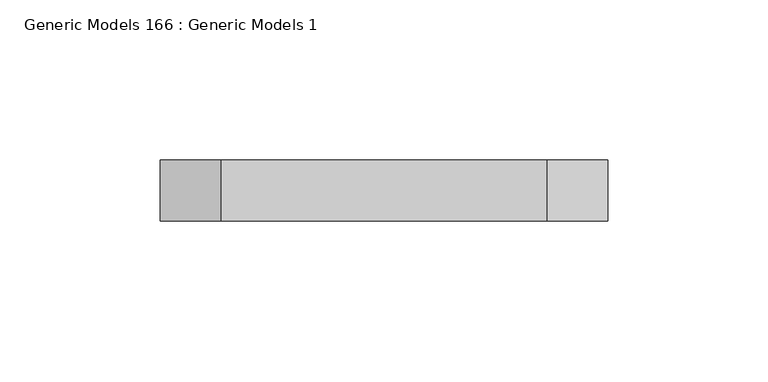
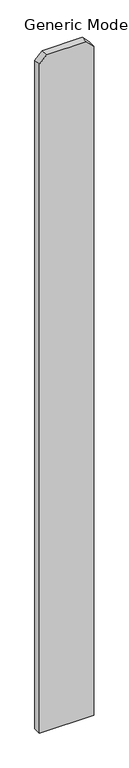
"""IFC4 building model written with IfcOpenShell, lengths in millimetres: proxy geometry, Generic Models 166 : Generic Models 1."""

from ifc_helpers import new_model, si_unit, frame, origin, place, context, project, spatial, polyline, outline, extrude, source, transform, mapped, element, save


def generic_models_166_generic_models_1_bb9aeded(model_context):
    return source(origin(), model_context, "Body", "SweptSolid", [
        extrude(outline(polyline([(76.2, 55294.2125), (1885.95, 55294.2125), (1905.0, 55275.1625), (1905.0, 55173.5625), (1885.95, 55154.5125), (76.2, 55154.5125), (76.2, 55294.2125)])), frame((0.0, 547.6875, 0.0), z_axis=(0.0, 1.0, 0.0), x_axis=(0.0, 0.0, 1.0)), (0.0, 0.0, 1.0), 19.05),
    ])


if __name__ == "__main__":
    model = new_model("IFC4")
    model_context = context("Model", 3, world=origin())
    ifc_project = project(units=[si_unit("LENGTHUNIT", "METRE", prefix="MILLI")], contexts=[model_context])
    site = spatial("IfcSite", under=ifc_project)
    building = spatial("IfcBuilding", under=site)
    placement = place(None, origin())
    generic_models_166_generic_models_1_shape = generic_models_166_generic_models_1_bb9aeded(model_context)
    element("IfcBuildingElementProxy", 1, Name="Generic Models 166 : Generic Models 1", ObjectType="Generic Models 166 : Generic Models 1", at=placement, inside=building, context=model_context, shape_type="MappedRepresentation", body=[
        mapped(generic_models_166_generic_models_1_shape, transform((0.0, 0.0, 0.0), x_axis=(1.0, 0.0, 0.0), y_axis=(0.0, 1.0, 0.0), z_axis=(0.0, 0.0, 1.0))),
    ])
    save(model, "model.ifc")

# Revit data of these elements
# Element 1 (IfcBuildingElementProxy, "Generic Models 166 : Generic Models 1")
#   Materials on its faces: "VERTICAL 1X6 CEDAR PLANKS W/ CLEAR WOOD SEALER"
# Materials
#   "VERTICAL 1X6 CEDAR PLANKS W/ CLEAR WOOD SEALER": class "Wood", colour RGB 234 198 147, transparency 0, Description = "Pinus Echinata", Cost = 0
